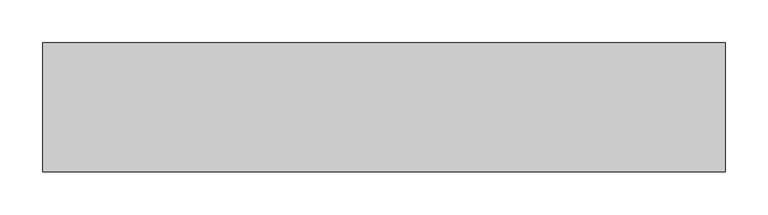
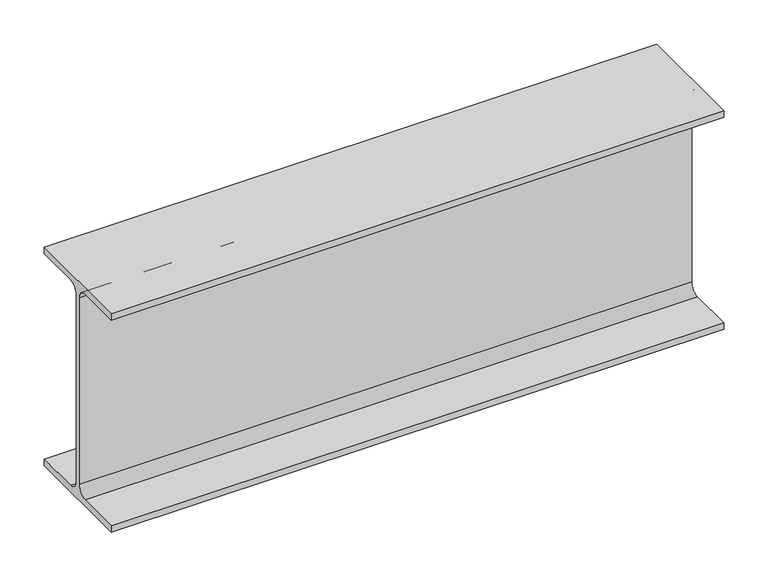
"""IFC4 building model written with IfcOpenShell, lengths in millimetres: beam geometry, 0912_Steel Framing_H-KSD3502 : H_SB_ASB_H-300x150x6.5x9."""

import ifcopenshell
import ifcopenshell.guid

model = None  # the IFC model being written
_history = None  # IfcOwnerHistory: only IFC2X3 demands one
_inside = {}  # id of a spatial element -> (the spatial element, [elements in it])
_under = {}  # id of a project, library or spatial element -> (it, [spatial elements below it])
_declared = {}  # id of a project -> (the project, [libraries it declares])
_typed = {}  # id of a type object -> (the type object, [elements of that type])
_made_of = {}  # id of a material, layer set ... -> (it, [elements and type objects made of it])


def new_model(schema):
    """Start an empty IFC model of exactly this schema.

    Asked for "IFC4X3", IfcOpenShell would pick the latest addendum, in which some entities
    have other attributes; the version numbers below select the first issue.
    IFC2X3 requires an IfcOwnerHistory on every rooted entity: one is made here for all.
    """
    global model, _history
    if schema == "IFC4X3":
        model = ifcopenshell.file(schema_version=(4, 3, 0, 0))
    else:
        model = ifcopenshell.file(schema=schema)
    _inside.clear()
    _under.clear()
    _declared.clear()
    _typed.clear()
    _made_of.clear()
    _history = None
    if model.schema == "IFC2X3":
        org = make("IfcOrganization", Name="unknown")
        user = make(
            "IfcPersonAndOrganization",
            ThePerson=make("IfcPerson", FamilyName="unknown"),
            TheOrganization=org,
        )
        app = make(
            "IfcApplication",
            ApplicationDeveloper=org,
            Version="unknown",
            ApplicationFullName="unknown",
            ApplicationIdentifier="unknown",
        )
        _history = make(
            "IfcOwnerHistory",
            OwningUser=user,
            OwningApplication=app,
            ChangeAction="ADDED",
            CreationDate=0,
        )
    return model


def make(cls, **values):
    """One entity of the class cls with the attributes given. An attribute that is None is left unset."""
    return model.create_entity(
        cls, **{name: value for name, value in values.items() if value is not None}
    )


def rooted(cls, **values):
    """An entity with a GlobalId (a new one), such as an element, a storey or a relation."""
    return make(cls, GlobalId=ifcopenshell.guid.new(), OwnerHistory=_history, **values)


def si_unit(unit_type, name, prefix=None):
    """IfcSIUnit, for example si_unit("LENGTHUNIT", "METRE", prefix="MILLI")."""
    return make("IfcSIUnit", UnitType=unit_type, Prefix=prefix, Name=name)


def assignment(units):
    """IfcUnitAssignment: the units of a project."""
    return None if units is None else make("IfcUnitAssignment", Units=units)


def point(xyz):
    """IfcCartesianPoint."""
    return None if xyz is None else make("IfcCartesianPoint", Coordinates=xyz)


def direction(xyz):
    """IfcDirection."""
    return None if xyz is None else make("IfcDirection", DirectionRatios=xyz)


def frame(location, z_axis=None, x_axis=None):
    """IfcAxis2Placement3D, a coordinate frame: its origin and axes. An axis left out is left unset."""
    return make(
        "IfcAxis2Placement3D",
        Location=point(location),
        Axis=direction(z_axis),
        RefDirection=direction(x_axis),
    )


def frame_2d(location, x_axis=None):
    """IfcAxis2Placement2D, a coordinate frame in the plane: its origin and x axis."""
    return make(
        "IfcAxis2Placement2D", Location=point(location), RefDirection=direction(x_axis)
    )


def origin():
    """The frame at (0, 0, 0) with its axes left unset."""
    return frame((0.0, 0.0, 0.0))


def place(relative_to, where):
    """IfcLocalPlacement: puts the frame where relative to a parent placement (None: the world)."""
    return make(
        "IfcLocalPlacement", PlacementRelTo=relative_to, RelativePlacement=where
    )


def context(
    kind, dimensions, precision=None, world=None, true_north=None, identifier=None
):
    """IfcGeometricRepresentationContext, for example the 3D "Model" context."""
    return make(
        "IfcGeometricRepresentationContext",
        ContextIdentifier=identifier,
        ContextType=kind,
        CoordinateSpaceDimension=dimensions,
        Precision=precision,
        WorldCoordinateSystem=world,
        TrueNorth=true_north,
    )


def project(units=None, contexts=None):
    """IfcProject with its units and contexts."""
    return rooted(
        "IfcProject",
        Name="project",
        RepresentationContexts=contexts,
        UnitsInContext=assignment(units),
    )


def spatial(cls, under=None, at=None, **own):
    """A site, building, storey or space (cls), placed at a placement, below another one or the project."""
    s = rooted(cls, ObjectPlacement=at, **own)
    if under is not None:
        _under.setdefault(under.id(), (under, []))[1].append(s)
    return s


def polyline(points):
    """IfcPolyline through the points."""
    return make("IfcPolyline", Points=[point(p) for p in points])


def circle_curve(where, radius):
    """IfcCircle in the frame where."""
    return make("IfcCircle", Position=where, Radius=radius)


def trimmed(basis, trim1, trim2, sense, master):
    """IfcTrimmedCurve: the piece of a basis curve between two trims."""
    return make(
        "IfcTrimmedCurve",
        BasisCurve=basis,
        Trim1=trim1,
        Trim2=trim2,
        SenseAgreement=sense,
        MasterRepresentation=master,
    )


def segment(curve, same_sense, transition):
    """IfcCompositeCurveSegment."""
    return make(
        "IfcCompositeCurveSegment",
        Transition=transition,
        SameSense=same_sense,
        ParentCurve=curve,
    )


def composite_curve(segments, self_intersect=None):
    """IfcCompositeCurve: segments joined end to end."""
    return make("IfcCompositeCurve", Segments=segments, SelfIntersect=self_intersect)


def outline(outer, holes=None, kind="AREA"):
    """IfcArbitraryClosedProfileDef: a profile drawn as a closed curve; with holes, ...WithVoids."""
    if holes is None:
        return make("IfcArbitraryClosedProfileDef", ProfileType=kind, OuterCurve=outer)
    return make(
        "IfcArbitraryProfileDefWithVoids",
        ProfileType=kind,
        OuterCurve=outer,
        InnerCurves=holes,
    )


def extrude(swept, where, along, depth):
    """IfcExtrudedAreaSolid: the profile swept, set in the frame where, extruded along a direction by depth."""
    return make(
        "IfcExtrudedAreaSolid",
        SweptArea=swept,
        Position=where,
        ExtrudedDirection=direction(along),
        Depth=depth,
    )


def shape(context_of_items, identifier, shape_type, items):
    """IfcShapeRepresentation: the items that make up one representation, for example the "Body"."""
    return make(
        "IfcShapeRepresentation",
        ContextOfItems=context_of_items,
        RepresentationIdentifier=identifier,
        RepresentationType=shape_type,
        Items=items,
    )


def source(mapping_origin, context_of_items, identifier, shape_type, items):
    """IfcRepresentationMap: a shape defined once, which mapped items show again and again."""
    return make(
        "IfcRepresentationMap",
        MappingOrigin=mapping_origin,
        MappedRepresentation=shape(context_of_items, identifier, shape_type, items),
    )


def transform(
    local_origin,
    x_axis=None,
    y_axis=None,
    z_axis=None,
    scale=None,
    scale2=None,
    scale3=None,
    uniform=True,
):
    """IfcCartesianTransformationOperator3D, or its non-uniform kind. x_axis, y_axis, z_axis: its Axis1, 2, 3."""
    if uniform:
        return make(
            "IfcCartesianTransformationOperator3D",
            Axis1=direction(x_axis),
            Axis2=direction(y_axis),
            LocalOrigin=point(local_origin),
            Scale=scale,
            Axis3=direction(z_axis),
        )
    return make(
        "IfcCartesianTransformationOperator3DnonUniform",
        Axis1=direction(x_axis),
        Axis2=direction(y_axis),
        LocalOrigin=point(local_origin),
        Scale=scale,
        Axis3=direction(z_axis),
        Scale2=scale2,
        Scale3=scale3,
    )


def mapped(mapping_source, mapping_target):
    """IfcMappedItem: shows the shape of a source again, moved by a transform."""
    return make(
        "IfcMappedItem", MappingSource=mapping_source, MappingTarget=mapping_target
    )


def made_of(thing, what):
    """Note that an element or type object is made of a material, layer set ...; save() writes the relation."""
    if what is not None:
        _made_of.setdefault(what.id(), (what, []))[1].append(thing)
    return thing


def element(
    cls,
    number,
    at=None,
    inside=None,
    cuts=None,
    type_object=None,
    material=None,
    context=None,
    identifier="Body",
    shape_type=None,
    held_by="IfcProductDefinitionShape",
    body=None,
    shapes=None,
    **own,
):
    """One element of the class cls, such as IfcWall. Its Tag is "e" and its number.

    at: its placement. inside: the storey or other place that contains it. cuts: it is an
    opening in that element (IfcRelVoidsElement). A single representation is given by context,
    identifier, shape_type and body (its items); several are given by shapes. held_by: the class
    of the entity that holds the representations. save() writes the other relations.
    """
    e = rooted(cls, Tag="e%d" % number, ObjectPlacement=at, **own)
    if body is not None:
        shapes = [shape(context, identifier, shape_type, body)]
    if shapes is not None:
        e.Representation = make(held_by, Representations=shapes)
    if inside is not None:
        _inside.setdefault(inside.id(), (inside, []))[1].append(e)
    if cuts is not None:
        rooted(
            "IfcRelVoidsElement", RelatingBuildingElement=cuts, RelatedOpeningElement=e
        )
    if type_object is not None:
        _typed.setdefault(type_object.id(), (type_object, []))[1].append(e)
    return made_of(e, material)


def aggregate(whole, parts):
    """IfcRelAggregates: a whole, such as a stair, and the parts it consists of."""
    return rooted("IfcRelAggregates", RelatingObject=whole, RelatedObjects=parts)


def save(model, path):
    """Write the relations noted so far, then the file.

    IfcRelAggregates (storeys below a building ...), IfcRelContainedInSpatialStructure (elements
    in a storey), IfcRelDefinesByType, IfcRelAssociatesMaterial and IfcRelDeclares: one each for
    every whole, place, type object, material and project.
    """
    for whole, parts in _under.values():
        aggregate(whole, parts)
    for where, things in _inside.values():
        rooted(
            "IfcRelContainedInSpatialStructure",
            RelatedElements=things,
            RelatingStructure=where,
        )
    for kind, things in _typed.values():
        rooted("IfcRelDefinesByType", RelatedObjects=things, RelatingType=kind)
    for what, things in _made_of.values():
        rooted("IfcRelAssociatesMaterial", RelatedObjects=things, RelatingMaterial=what)
    for by, libraries in _declared.values():
        rooted("IfcRelDeclares", RelatingContext=by, RelatedDefinitions=libraries)
    model.write(path)


def beam_e2def3fa(model_context):
    return source(origin(), model_context, "Body", "SweptSolid", [
        extrude(outline(composite_curve([segment(polyline([(75.0, -141.0), (75.0, -150.0), (-75.0, -150.0), (-75.0, -141.0), (-16.25, -141.0)]), True, "CONTINUOUS"), segment(trimmed(circle_curve(frame_2d((-16.25, -128.0)), 13.0), [point((-16.25, -141.0))], [point((-3.25, -128.0))], True, "CARTESIAN"), True, "CONTINUOUS"), segment(polyline([(-3.25, -128.0), (-3.25, 128.0)]), True, "CONTINUOUS"), segment(trimmed(circle_curve(frame_2d((-16.25, 128.0)), 13.0), [point((-3.25, 128.0))], [point((-16.25, 141.0))], True, "CARTESIAN"), True, "CONTINUOUS"), segment(polyline([(-16.25, 141.0), (-75.0, 141.0), (-75.0, 150.0), (75.0, 150.0), (75.0, 141.0), (16.25, 141.0)]), True, "CONTINUOUS"), segment(trimmed(circle_curve(frame_2d((16.25, 128.0)), 13.0), [point((16.25, 141.0))], [point((3.25, 128.0))], True, "CARTESIAN"), True, "CONTINUOUS"), segment(polyline([(3.25, 128.0), (3.25, -128.0)]), True, "CONTINUOUS"), segment(trimmed(circle_curve(frame_2d((16.25, -128.0)), 13.0), [point((3.25, -128.0))], [point((16.25, -141.0))], True, "CARTESIAN"), True, "CONTINUOUS"), segment(polyline([(16.25, -141.0), (75.0, -141.0)]), True, "CONTINUOUS")], self_intersect=False)), frame((-445.0, 0.0, 0.0), z_axis=(1.0, 0.0, 0.0), x_axis=(0.0, 1.0, 0.0)), (0.0, 0.0, 1.0), 794.8),
    ])


if __name__ == "__main__":
    model = new_model("IFC4")
    model_context = context("Model", 3, world=origin())
    ifc_project = project(units=[si_unit("LENGTHUNIT", "METRE", prefix="MILLI")], contexts=[model_context])
    site = spatial("IfcSite", under=ifc_project)
    building = spatial("IfcBuilding", under=site)
    placement = place(None, origin())
    beam_shape = beam_e2def3fa(model_context)
    element("IfcBeam", 1, ObjectType="0912_Steel Framing_H-KSD3502 : H_SB_ASB_H-300x150x6.5x9", at=placement, inside=building, context=model_context, shape_type="MappedRepresentation", body=[
        mapped(beam_shape, transform((0.0, 0.0, 0.0), x_axis=(1.0, 0.0, 0.0), y_axis=(0.0, 1.0, 0.0), z_axis=(0.0, 0.0, 1.0))),
    ])
    save(model, "model.ifc")

# Revit data of these elements
# Type "0912_Steel Framing_H-KSD3502 : H_SB_ASB_H-300x150x6.5x9"
#   H_WM Code_1 = "S01AA002-00001 | Main Steel Structure Fabrication Work | Shelter/Building | Medium Steel - Standard (90KG/M>Weight≥30KG/M) | Material: (   )"
#   H_WM Code_2 = "S03AA028-00001 | Main Steel Structure Erection Work | Shelter/Building | Medium Steel (90KG/M>Weight≥30KG/M) | Material: (   )"
#   H_WM Code_3 = "S01AA010-00001 | Main Steel Structure Fabrication Work | Shelter/Building | Steel Painting/Coating | for Non-Fireproofed Steel Surface, Surface Preparation, Primer, Second & Final Coat | Material: (   )"
#   H_Q'ty Cal Type Tag = "SB-Q2"
#   Width = 15.0 cm
#   Web Thickness = 0.65 cm
#   Web Fillet = 1.3 cm
#   Warping Constant = 107000.0 cm⁶
#   W = 0
#   Torsional Moment of Inertia = 9.9539 cm⁴
#   Section Area = 46.78 cm²
#   Plastic Modulus weak axis = 105.0 cm³
#   Plastic Modulus strong axis = 542.0 cm³
#   Perimeter = 1.17 m²/m
#   Nominal Weight = 36.70 kgf/m
#   Moment of Inertia weak axis = 508.00 cm⁴
#   Moment of Inertia strong axis = 7210.00 cm⁴
#   Height = 30.0 cm
#   Flange Thickness = 0.9 cm
#   Elastic Modulus weak axis = 67.7 cm³
#   Elastic Modulus strong axis = 481.0 cm³
#   Centroid Vertical = 15.0 cm
#   Centroid Horizontal = 7.5 cm
#   Ix = 72100000
#   Length [instance default] = 1.5240 m
#   Zx = 542000
#   b = 0.1500 m
#   h = 0.3000 m
#   r = 0.0130 m
#   s = 0.0065 m
#   t = 0.0090 m
#   A = 0.004678 m²
#   Structural Material [instance default] = Steel, 45-345
#   Assembly Code = ""
# Element 1 (IfcBeam, "0912_Steel Framing_H-KSD3502 : H_SB_ASB_H-300x150x6.5x9")
#   Structural Material = none
# Materials
#   "Steel, 45-345": class "Metal", colour RGB 189 187 185, transparency 0, Description = "Steel 345 MPa", Cost = 0
